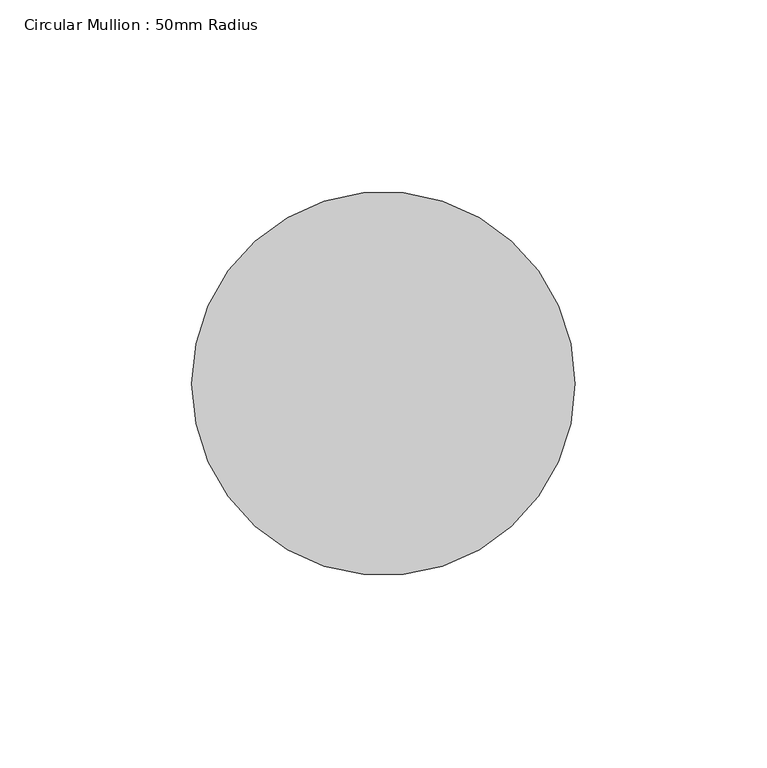
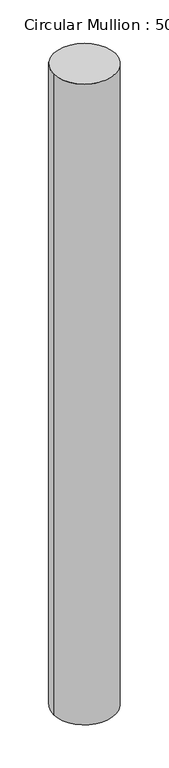
"""IFC4 building model written with IfcOpenShell, lengths in millimetres: member geometry, Circular Mullion : 50mm Radius."""

import ifcopenshell
import ifcopenshell.guid

model = None  # the IFC model being written
_history = None  # IfcOwnerHistory: only IFC2X3 demands one
_inside = {}  # id of a spatial element -> (the spatial element, [elements in it])
_under = {}  # id of a project, library or spatial element -> (it, [spatial elements below it])
_declared = {}  # id of a project -> (the project, [libraries it declares])
_typed = {}  # id of a type object -> (the type object, [elements of that type])
_made_of = {}  # id of a material, layer set ... -> (it, [elements and type objects made of it])


def new_model(schema):
    """Start an empty IFC model of exactly this schema.

    Asked for "IFC4X3", IfcOpenShell would pick the latest addendum, in which some entities
    have other attributes; the version numbers below select the first issue.
    IFC2X3 requires an IfcOwnerHistory on every rooted entity: one is made here for all.
    """
    global model, _history
    if schema == "IFC4X3":
        model = ifcopenshell.file(schema_version=(4, 3, 0, 0))
    else:
        model = ifcopenshell.file(schema=schema)
    _inside.clear()
    _under.clear()
    _declared.clear()
    _typed.clear()
    _made_of.clear()
    _history = None
    if model.schema == "IFC2X3":
        org = make("IfcOrganization", Name="unknown")
        user = make(
            "IfcPersonAndOrganization",
            ThePerson=make("IfcPerson", FamilyName="unknown"),
            TheOrganization=org,
        )
        app = make(
            "IfcApplication",
            ApplicationDeveloper=org,
            Version="unknown",
            ApplicationFullName="unknown",
            ApplicationIdentifier="unknown",
        )
        _history = make(
            "IfcOwnerHistory",
            OwningUser=user,
            OwningApplication=app,
            ChangeAction="ADDED",
            CreationDate=0,
        )
    return model


def make(cls, **values):
    """One entity of the class cls with the attributes given. An attribute that is None is left unset."""
    return model.create_entity(
        cls, **{name: value for name, value in values.items() if value is not None}
    )


def rooted(cls, **values):
    """An entity with a GlobalId (a new one), such as an element, a storey or a relation."""
    return make(cls, GlobalId=ifcopenshell.guid.new(), OwnerHistory=_history, **values)


def si_unit(unit_type, name, prefix=None):
    """IfcSIUnit, for example si_unit("LENGTHUNIT", "METRE", prefix="MILLI")."""
    return make("IfcSIUnit", UnitType=unit_type, Prefix=prefix, Name=name)


def assignment(units):
    """IfcUnitAssignment: the units of a project."""
    return None if units is None else make("IfcUnitAssignment", Units=units)


def point(xyz):
    """IfcCartesianPoint."""
    return None if xyz is None else make("IfcCartesianPoint", Coordinates=xyz)


def direction(xyz):
    """IfcDirection."""
    return None if xyz is None else make("IfcDirection", DirectionRatios=xyz)


def frame(location, z_axis=None, x_axis=None):
    """IfcAxis2Placement3D, a coordinate frame: its origin and axes. An axis left out is left unset."""
    return make(
        "IfcAxis2Placement3D",
        Location=point(location),
        Axis=direction(z_axis),
        RefDirection=direction(x_axis),
    )


def frame_2d(location, x_axis=None):
    """IfcAxis2Placement2D, a coordinate frame in the plane: its origin and x axis."""
    return make(
        "IfcAxis2Placement2D", Location=point(location), RefDirection=direction(x_axis)
    )


def origin():
    """The frame at (0, 0, 0) with its axes left unset."""
    return frame((0.0, 0.0, 0.0))


def origin_2d():
    """The frame at (0, 0) in the plane with its x axis left unset."""
    return frame_2d((0.0, 0.0))


def place(relative_to, where):
    """IfcLocalPlacement: puts the frame where relative to a parent placement (None: the world)."""
    return make(
        "IfcLocalPlacement", PlacementRelTo=relative_to, RelativePlacement=where
    )


def context(
    kind, dimensions, precision=None, world=None, true_north=None, identifier=None
):
    """IfcGeometricRepresentationContext, for example the 3D "Model" context."""
    return make(
        "IfcGeometricRepresentationContext",
        ContextIdentifier=identifier,
        ContextType=kind,
        CoordinateSpaceDimension=dimensions,
        Precision=precision,
        WorldCoordinateSystem=world,
        TrueNorth=true_north,
    )


def project(units=None, contexts=None):
    """IfcProject with its units and contexts."""
    return rooted(
        "IfcProject",
        Name="project",
        RepresentationContexts=contexts,
        UnitsInContext=assignment(units),
    )


def spatial(cls, under=None, at=None, **own):
    """A site, building, storey or space (cls), placed at a placement, below another one or the project."""
    s = rooted(cls, ObjectPlacement=at, **own)
    if under is not None:
        _under.setdefault(under.id(), (under, []))[1].append(s)
    return s


def circle_curve(where, radius):
    """IfcCircle in the frame where."""
    return make("IfcCircle", Position=where, Radius=radius)


def trimmed(basis, trim1, trim2, sense, master):
    """IfcTrimmedCurve: the piece of a basis curve between two trims."""
    return make(
        "IfcTrimmedCurve",
        BasisCurve=basis,
        Trim1=trim1,
        Trim2=trim2,
        SenseAgreement=sense,
        MasterRepresentation=master,
    )


def segment(curve, same_sense, transition):
    """IfcCompositeCurveSegment."""
    return make(
        "IfcCompositeCurveSegment",
        Transition=transition,
        SameSense=same_sense,
        ParentCurve=curve,
    )


def composite_curve(segments, self_intersect=None):
    """IfcCompositeCurve: segments joined end to end."""
    return make("IfcCompositeCurve", Segments=segments, SelfIntersect=self_intersect)


def outline(outer, holes=None, kind="AREA"):
    """IfcArbitraryClosedProfileDef: a profile drawn as a closed curve; with holes, ...WithVoids."""
    if holes is None:
        return make("IfcArbitraryClosedProfileDef", ProfileType=kind, OuterCurve=outer)
    return make(
        "IfcArbitraryProfileDefWithVoids",
        ProfileType=kind,
        OuterCurve=outer,
        InnerCurves=holes,
    )


def extrude(swept, where, along, depth):
    """IfcExtrudedAreaSolid: the profile swept, set in the frame where, extruded along a direction by depth."""
    return make(
        "IfcExtrudedAreaSolid",
        SweptArea=swept,
        Position=where,
        ExtrudedDirection=direction(along),
        Depth=depth,
    )


def shape(context_of_items, identifier, shape_type, items):
    """IfcShapeRepresentation: the items that make up one representation, for example the "Body"."""
    return make(
        "IfcShapeRepresentation",
        ContextOfItems=context_of_items,
        RepresentationIdentifier=identifier,
        RepresentationType=shape_type,
        Items=items,
    )


def source(mapping_origin, context_of_items, identifier, shape_type, items):
    """IfcRepresentationMap: a shape defined once, which mapped items show again and again."""
    return make(
        "IfcRepresentationMap",
        MappingOrigin=mapping_origin,
        MappedRepresentation=shape(context_of_items, identifier, shape_type, items),
    )


def transform(
    local_origin,
    x_axis=None,
    y_axis=None,
    z_axis=None,
    scale=None,
    scale2=None,
    scale3=None,
    uniform=True,
):
    """IfcCartesianTransformationOperator3D, or its non-uniform kind. x_axis, y_axis, z_axis: its Axis1, 2, 3."""
    if uniform:
        return make(
            "IfcCartesianTransformationOperator3D",
            Axis1=direction(x_axis),
            Axis2=direction(y_axis),
            LocalOrigin=point(local_origin),
            Scale=scale,
            Axis3=direction(z_axis),
        )
    return make(
        "IfcCartesianTransformationOperator3DnonUniform",
        Axis1=direction(x_axis),
        Axis2=direction(y_axis),
        LocalOrigin=point(local_origin),
        Scale=scale,
        Axis3=direction(z_axis),
        Scale2=scale2,
        Scale3=scale3,
    )


def mapped(mapping_source, mapping_target):
    """IfcMappedItem: shows the shape of a source again, moved by a transform."""
    return make(
        "IfcMappedItem", MappingSource=mapping_source, MappingTarget=mapping_target
    )


def made_of(thing, what):
    """Note that an element or type object is made of a material, layer set ...; save() writes the relation."""
    if what is not None:
        _made_of.setdefault(what.id(), (what, []))[1].append(thing)
    return thing


def element(
    cls,
    number,
    at=None,
    inside=None,
    cuts=None,
    type_object=None,
    material=None,
    context=None,
    identifier="Body",
    shape_type=None,
    held_by="IfcProductDefinitionShape",
    body=None,
    shapes=None,
    **own,
):
    """One element of the class cls, such as IfcWall. Its Tag is "e" and its number.

    at: its placement. inside: the storey or other place that contains it. cuts: it is an
    opening in that element (IfcRelVoidsElement). A single representation is given by context,
    identifier, shape_type and body (its items); several are given by shapes. held_by: the class
    of the entity that holds the representations. save() writes the other relations.
    """
    e = rooted(cls, Tag="e%d" % number, ObjectPlacement=at, **own)
    if body is not None:
        shapes = [shape(context, identifier, shape_type, body)]
    if shapes is not None:
        e.Representation = make(held_by, Representations=shapes)
    if inside is not None:
        _inside.setdefault(inside.id(), (inside, []))[1].append(e)
    if cuts is not None:
        rooted(
            "IfcRelVoidsElement", RelatingBuildingElement=cuts, RelatedOpeningElement=e
        )
    if type_object is not None:
        _typed.setdefault(type_object.id(), (type_object, []))[1].append(e)
    return made_of(e, material)


def aggregate(whole, parts):
    """IfcRelAggregates: a whole, such as a stair, and the parts it consists of."""
    return rooted("IfcRelAggregates", RelatingObject=whole, RelatedObjects=parts)


def save(model, path):
    """Write the relations noted so far, then the file.

    IfcRelAggregates (storeys below a building ...), IfcRelContainedInSpatialStructure (elements
    in a storey), IfcRelDefinesByType, IfcRelAssociatesMaterial and IfcRelDeclares: one each for
    every whole, place, type object, material and project.
    """
    for whole, parts in _under.values():
        aggregate(whole, parts)
    for where, things in _inside.values():
        rooted(
            "IfcRelContainedInSpatialStructure",
            RelatedElements=things,
            RelatingStructure=where,
        )
    for kind, things in _typed.values():
        rooted("IfcRelDefinesByType", RelatedObjects=things, RelatingType=kind)
    for what, things in _made_of.values():
        rooted("IfcRelAssociatesMaterial", RelatedObjects=things, RelatingMaterial=what)
    for by, libraries in _declared.values():
        rooted("IfcRelDeclares", RelatingContext=by, RelatedDefinitions=libraries)
    model.write(path)


def circular_mullion_50mm_radius_52fda331(model_context):
    return source(origin(), model_context, "Body", "SweptSolid", [
        extrude(outline(composite_curve([segment(trimmed(circle_curve(origin_2d(), 50.0), [point((50.0, 0.0))], [point((-50.0, 0.0))], False, "CARTESIAN"), True, "CONTINUOUS"), segment(trimmed(circle_curve(origin_2d(), 50.0), [point((-50.0, 0.0))], [point((50.0, 0.0))], False, "CARTESIAN"), True, "CONTINUOUS")], self_intersect=False)), frame((0.0, 0.0, -1093.9160949), z_axis=(0.0, 0.0, 1.0), x_axis=(1.0, 0.0, 0.0)), (0.0, 0.0, 1.0), 1093.9160949),
    ])


if __name__ == "__main__":
    model = new_model("IFC4")
    model_context = context("Model", 3, world=origin())
    ifc_project = project(units=[si_unit("LENGTHUNIT", "METRE", prefix="MILLI")], contexts=[model_context])
    site = spatial("IfcSite", under=ifc_project)
    building = spatial("IfcBuilding", under=site)
    placement = place(None, origin())
    circular_mullion_50mm_radius_shape = circular_mullion_50mm_radius_52fda331(model_context)
    element("IfcMember", 1, ObjectType="Circular Mullion : 50mm Radius", at=placement, inside=building, context=model_context, shape_type="MappedRepresentation", body=[
        mapped(circular_mullion_50mm_radius_shape, transform((0.0, 0.0, 0.0), x_axis=(1.0, 0.0, 0.0), y_axis=(0.0, 1.0, 0.0), z_axis=(0.0, 0.0, 1.0))),
    ])
    save(model, "model.ifc")

# Revit data of these elements
# Type "Circular Mullion : 50mm Radius"
#   built-in parameter 1007350 = 0.164042 (stored number, unit not read)
# Element 1 (IfcMember, "Circular Mullion : 50mm Radius")
#   Materials on its faces: "Aluminium"
# Materials
#   "Aluminium": class "Metal", colour RGB 247 247 247, transparency 0, Description = "Aluminium 6061", Cost = 0
